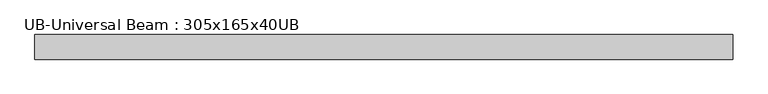
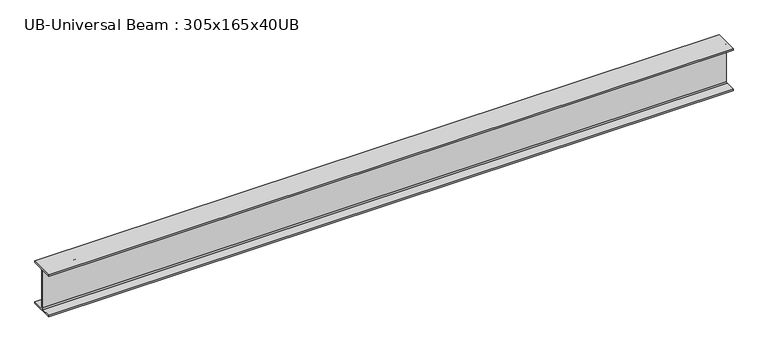
"""IFC4 building model written with IfcOpenShell, lengths in millimetres: beam geometry, UB-Universal Beam : 305x165x40UB."""

import ifcopenshell
import ifcopenshell.guid

model = None  # the IFC model being written
_history = None  # IfcOwnerHistory: only IFC2X3 demands one
_inside = {}  # id of a spatial element -> (the spatial element, [elements in it])
_under = {}  # id of a project, library or spatial element -> (it, [spatial elements below it])
_declared = {}  # id of a project -> (the project, [libraries it declares])
_typed = {}  # id of a type object -> (the type object, [elements of that type])
_made_of = {}  # id of a material, layer set ... -> (it, [elements and type objects made of it])


def new_model(schema):
    """Start an empty IFC model of exactly this schema.

    Asked for "IFC4X3", IfcOpenShell would pick the latest addendum, in which some entities
    have other attributes; the version numbers below select the first issue.
    IFC2X3 requires an IfcOwnerHistory on every rooted entity: one is made here for all.
    """
    global model, _history
    if schema == "IFC4X3":
        model = ifcopenshell.file(schema_version=(4, 3, 0, 0))
    else:
        model = ifcopenshell.file(schema=schema)
    _inside.clear()
    _under.clear()
    _declared.clear()
    _typed.clear()
    _made_of.clear()
    _history = None
    if model.schema == "IFC2X3":
        org = make("IfcOrganization", Name="unknown")
        user = make(
            "IfcPersonAndOrganization",
            ThePerson=make("IfcPerson", FamilyName="unknown"),
            TheOrganization=org,
        )
        app = make(
            "IfcApplication",
            ApplicationDeveloper=org,
            Version="unknown",
            ApplicationFullName="unknown",
            ApplicationIdentifier="unknown",
        )
        _history = make(
            "IfcOwnerHistory",
            OwningUser=user,
            OwningApplication=app,
            ChangeAction="ADDED",
            CreationDate=0,
        )
    return model


def make(cls, **values):
    """One entity of the class cls with the attributes given. An attribute that is None is left unset."""
    return model.create_entity(
        cls, **{name: value for name, value in values.items() if value is not None}
    )


def rooted(cls, **values):
    """An entity with a GlobalId (a new one), such as an element, a storey or a relation."""
    return make(cls, GlobalId=ifcopenshell.guid.new(), OwnerHistory=_history, **values)


def si_unit(unit_type, name, prefix=None):
    """IfcSIUnit, for example si_unit("LENGTHUNIT", "METRE", prefix="MILLI")."""
    return make("IfcSIUnit", UnitType=unit_type, Prefix=prefix, Name=name)


def assignment(units):
    """IfcUnitAssignment: the units of a project."""
    return None if units is None else make("IfcUnitAssignment", Units=units)


def point(xyz):
    """IfcCartesianPoint."""
    return None if xyz is None else make("IfcCartesianPoint", Coordinates=xyz)


def direction(xyz):
    """IfcDirection."""
    return None if xyz is None else make("IfcDirection", DirectionRatios=xyz)


def frame(location, z_axis=None, x_axis=None):
    """IfcAxis2Placement3D, a coordinate frame: its origin and axes. An axis left out is left unset."""
    return make(
        "IfcAxis2Placement3D",
        Location=point(location),
        Axis=direction(z_axis),
        RefDirection=direction(x_axis),
    )


def frame_2d(location, x_axis=None):
    """IfcAxis2Placement2D, a coordinate frame in the plane: its origin and x axis."""
    return make(
        "IfcAxis2Placement2D", Location=point(location), RefDirection=direction(x_axis)
    )


def origin():
    """The frame at (0, 0, 0) with its axes left unset."""
    return frame((0.0, 0.0, 0.0))


def place(relative_to, where):
    """IfcLocalPlacement: puts the frame where relative to a parent placement (None: the world)."""
    return make(
        "IfcLocalPlacement", PlacementRelTo=relative_to, RelativePlacement=where
    )


def context(
    kind, dimensions, precision=None, world=None, true_north=None, identifier=None
):
    """IfcGeometricRepresentationContext, for example the 3D "Model" context."""
    return make(
        "IfcGeometricRepresentationContext",
        ContextIdentifier=identifier,
        ContextType=kind,
        CoordinateSpaceDimension=dimensions,
        Precision=precision,
        WorldCoordinateSystem=world,
        TrueNorth=true_north,
    )


def project(units=None, contexts=None):
    """IfcProject with its units and contexts."""
    return rooted(
        "IfcProject",
        Name="project",
        RepresentationContexts=contexts,
        UnitsInContext=assignment(units),
    )


def spatial(cls, under=None, at=None, **own):
    """A site, building, storey or space (cls), placed at a placement, below another one or the project."""
    s = rooted(cls, ObjectPlacement=at, **own)
    if under is not None:
        _under.setdefault(under.id(), (under, []))[1].append(s)
    return s


def polyline(points):
    """IfcPolyline through the points."""
    return make("IfcPolyline", Points=[point(p) for p in points])


def circle_curve(where, radius):
    """IfcCircle in the frame where."""
    return make("IfcCircle", Position=where, Radius=radius)


def trimmed(basis, trim1, trim2, sense, master):
    """IfcTrimmedCurve: the piece of a basis curve between two trims."""
    return make(
        "IfcTrimmedCurve",
        BasisCurve=basis,
        Trim1=trim1,
        Trim2=trim2,
        SenseAgreement=sense,
        MasterRepresentation=master,
    )


def segment(curve, same_sense, transition):
    """IfcCompositeCurveSegment."""
    return make(
        "IfcCompositeCurveSegment",
        Transition=transition,
        SameSense=same_sense,
        ParentCurve=curve,
    )


def composite_curve(segments, self_intersect=None):
    """IfcCompositeCurve: segments joined end to end."""
    return make("IfcCompositeCurve", Segments=segments, SelfIntersect=self_intersect)


def outline(outer, holes=None, kind="AREA"):
    """IfcArbitraryClosedProfileDef: a profile drawn as a closed curve; with holes, ...WithVoids."""
    if holes is None:
        return make("IfcArbitraryClosedProfileDef", ProfileType=kind, OuterCurve=outer)
    return make(
        "IfcArbitraryProfileDefWithVoids",
        ProfileType=kind,
        OuterCurve=outer,
        InnerCurves=holes,
    )


def extrude(swept, where, along, depth):
    """IfcExtrudedAreaSolid: the profile swept, set in the frame where, extruded along a direction by depth."""
    return make(
        "IfcExtrudedAreaSolid",
        SweptArea=swept,
        Position=where,
        ExtrudedDirection=direction(along),
        Depth=depth,
    )


def shape(context_of_items, identifier, shape_type, items):
    """IfcShapeRepresentation: the items that make up one representation, for example the "Body"."""
    return make(
        "IfcShapeRepresentation",
        ContextOfItems=context_of_items,
        RepresentationIdentifier=identifier,
        RepresentationType=shape_type,
        Items=items,
    )


def source(mapping_origin, context_of_items, identifier, shape_type, items):
    """IfcRepresentationMap: a shape defined once, which mapped items show again and again."""
    return make(
        "IfcRepresentationMap",
        MappingOrigin=mapping_origin,
        MappedRepresentation=shape(context_of_items, identifier, shape_type, items),
    )


def transform(
    local_origin,
    x_axis=None,
    y_axis=None,
    z_axis=None,
    scale=None,
    scale2=None,
    scale3=None,
    uniform=True,
):
    """IfcCartesianTransformationOperator3D, or its non-uniform kind. x_axis, y_axis, z_axis: its Axis1, 2, 3."""
    if uniform:
        return make(
            "IfcCartesianTransformationOperator3D",
            Axis1=direction(x_axis),
            Axis2=direction(y_axis),
            LocalOrigin=point(local_origin),
            Scale=scale,
            Axis3=direction(z_axis),
        )
    return make(
        "IfcCartesianTransformationOperator3DnonUniform",
        Axis1=direction(x_axis),
        Axis2=direction(y_axis),
        LocalOrigin=point(local_origin),
        Scale=scale,
        Axis3=direction(z_axis),
        Scale2=scale2,
        Scale3=scale3,
    )


def mapped(mapping_source, mapping_target):
    """IfcMappedItem: shows the shape of a source again, moved by a transform."""
    return make(
        "IfcMappedItem", MappingSource=mapping_source, MappingTarget=mapping_target
    )


def made_of(thing, what):
    """Note that an element or type object is made of a material, layer set ...; save() writes the relation."""
    if what is not None:
        _made_of.setdefault(what.id(), (what, []))[1].append(thing)
    return thing


def element(
    cls,
    number,
    at=None,
    inside=None,
    cuts=None,
    type_object=None,
    material=None,
    context=None,
    identifier="Body",
    shape_type=None,
    held_by="IfcProductDefinitionShape",
    body=None,
    shapes=None,
    **own,
):
    """One element of the class cls, such as IfcWall. Its Tag is "e" and its number.

    at: its placement. inside: the storey or other place that contains it. cuts: it is an
    opening in that element (IfcRelVoidsElement). A single representation is given by context,
    identifier, shape_type and body (its items); several are given by shapes. held_by: the class
    of the entity that holds the representations. save() writes the other relations.
    """
    e = rooted(cls, Tag="e%d" % number, ObjectPlacement=at, **own)
    if body is not None:
        shapes = [shape(context, identifier, shape_type, body)]
    if shapes is not None:
        e.Representation = make(held_by, Representations=shapes)
    if inside is not None:
        _inside.setdefault(inside.id(), (inside, []))[1].append(e)
    if cuts is not None:
        rooted(
            "IfcRelVoidsElement", RelatingBuildingElement=cuts, RelatedOpeningElement=e
        )
    if type_object is not None:
        _typed.setdefault(type_object.id(), (type_object, []))[1].append(e)
    return made_of(e, material)


def aggregate(whole, parts):
    """IfcRelAggregates: a whole, such as a stair, and the parts it consists of."""
    return rooted("IfcRelAggregates", RelatingObject=whole, RelatedObjects=parts)


def save(model, path):
    """Write the relations noted so far, then the file.

    IfcRelAggregates (storeys below a building ...), IfcRelContainedInSpatialStructure (elements
    in a storey), IfcRelDefinesByType, IfcRelAssociatesMaterial and IfcRelDeclares: one each for
    every whole, place, type object, material and project.
    """
    for whole, parts in _under.values():
        aggregate(whole, parts)
    for where, things in _inside.values():
        rooted(
            "IfcRelContainedInSpatialStructure",
            RelatedElements=things,
            RelatingStructure=where,
        )
    for kind, things in _typed.values():
        rooted("IfcRelDefinesByType", RelatedObjects=things, RelatingType=kind)
    for what, things in _made_of.values():
        rooted("IfcRelAssociatesMaterial", RelatedObjects=things, RelatingMaterial=what)
    for by, libraries in _declared.values():
        rooted("IfcRelDeclares", RelatingContext=by, RelatedDefinitions=libraries)
    model.write(path)


def ub_universal_beam_305x165x40ub_4e97a9be(model_context):
    return source(origin(), model_context, "Body", "SweptSolid", [
        extrude(outline(composite_curve([segment(polyline([(82.5, -141.5), (82.5, -151.7), (-82.5, -151.7), (-82.5, -141.5), (-11.9, -141.5)]), True, "CONTINUOUS"), segment(trimmed(circle_curve(frame_2d((-11.9, -132.6)), 8.9), [point((-11.9, -141.5))], [point((-3.0, -132.6))], True, "CARTESIAN"), True, "CONTINUOUS"), segment(polyline([(-3.0, -132.6), (-3.0, 132.6)]), True, "CONTINUOUS"), segment(trimmed(circle_curve(frame_2d((-11.9, 132.6)), 8.9), [point((-3.0, 132.6))], [point((-11.9, 141.5))], True, "CARTESIAN"), True, "CONTINUOUS"), segment(polyline([(-11.9, 141.5), (-82.5, 141.5), (-82.5, 151.7), (82.5, 151.7), (82.5, 141.5), (11.9, 141.5)]), True, "CONTINUOUS"), segment(trimmed(circle_curve(frame_2d((11.9, 132.6)), 8.9), [point((11.9, 141.5))], [point((3.0, 132.6))], True, "CARTESIAN"), True, "CONTINUOUS"), segment(polyline([(3.0, 132.6), (3.0, -132.6)]), True, "CONTINUOUS"), segment(trimmed(circle_curve(frame_2d((11.9, -132.6)), 8.9), [point((3.0, -132.6))], [point((11.9, -141.5))], True, "CARTESIAN"), True, "CONTINUOUS"), segment(polyline([(11.9, -141.5), (82.5, -141.5)]), True, "CONTINUOUS")], self_intersect=False)), frame((-2334.65, 0.0, 0.0), z_axis=(1.0, 0.0, 0.0), x_axis=(0.0, 1.0, 0.0)), (0.0, 0.0, 1.0), 4669.3),
    ])


if __name__ == "__main__":
    model = new_model("IFC4")
    model_context = context("Model", 3, world=origin())
    ifc_project = project(units=[si_unit("LENGTHUNIT", "METRE", prefix="MILLI")], contexts=[model_context])
    site = spatial("IfcSite", under=ifc_project)
    building = spatial("IfcBuilding", under=site)
    placement = place(None, origin())
    ub_universal_beam_305x165x40ub_shape = ub_universal_beam_305x165x40ub_4e97a9be(model_context)
    element("IfcBeam", 1, ObjectType="UB-Universal Beam : 305x165x40UB", at=placement, inside=building, context=model_context, shape_type="MappedRepresentation", body=[
        mapped(ub_universal_beam_305x165x40ub_shape, transform((0.0, 0.0, 0.0), x_axis=(1.0, 0.0, 0.0), y_axis=(0.0, 1.0, 0.0), z_axis=(0.0, 0.0, 1.0))),
    ])
    save(model, "model.ifc")

# Revit data of these elements
# Type "UB-Universal Beam : 305x165x40UB"
#   Nominal h = "305"
#   W = 0
#   Start Extension Calculation [instance default] = 3000 mm
#   Start Extension [instance default] = -12.7 mm
#   End Extension Calculation [instance default] = 3000 mm
#   End Extension [instance default] = -12.7 mm
#   Ix = 8503
#   Length [instance default] = 1524 mm
#   M = 40.3
#   Zx = 560
#   b = 165 mm
#   h = 303.4 mm
#   r = 8.9 mm
#   s = 6 mm
#   t = 10.2 mm
#   A = 0.005 m²
#   Structural Material [instance default] = Metal - Steel - 345 MPa
#   Assembly Code = ""
# Element 1 (IfcBeam, "UB-Universal Beam : 305x165x40UB")
#   Materials on its faces: "Metal - Steel - 345 MPa"
# Materials
#   "Metal - Steel - 345 MPa": class "Metal", colour RGB 241 46 46, transparency 0
